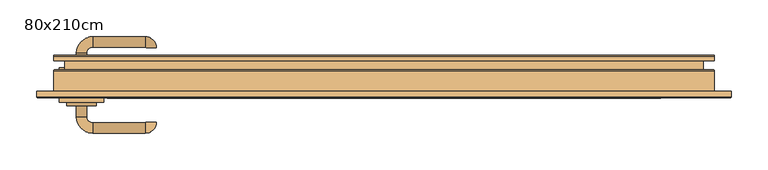
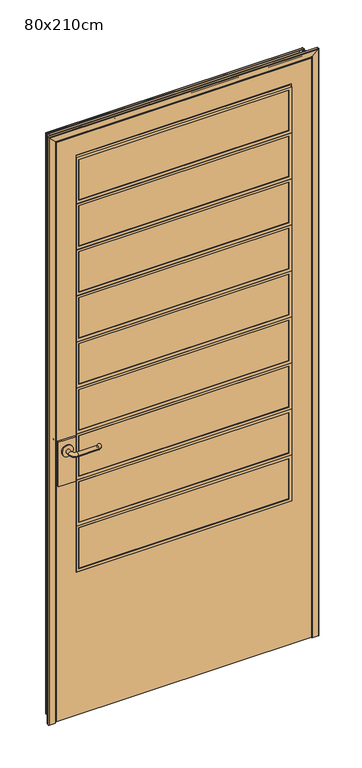
"""IFC4 building model written with IfcOpenShell, lengths in millimetres: door geometry, Porta de Abrir Metálica com Divisões Horizontais : 80x210cm."""

from ifc_helpers import new_model, si_unit, point, frame, frame_2d, origin, place, context, project, spatial, polyline, circle_curve, ellipse_curve, trimmed, segment, composite_curve, outline, extrude, source, transform, mapped, element, save
from ifc_brep_helpers import plane_surface, cylinder_surface, revolved_surface, advanced_brep


def door_80x210cm_38478dd2(model_context):
    return source(origin(), model_context, "Body", "SolidModel", [
        extrude(outline(polyline([(367.0, -87.5), (367.0, -92.5), (-367.0, -92.5), (-367.0, -87.5), (367.0, -87.5)])), frame((0.0, 0.0, 1955.6666667), z_axis=(0.0, 0.0, 1.0), x_axis=(1.0, 0.0, 0.0)), (0.0, 0.0, 1.0), 150.0),
        extrude(outline(polyline([(1945.6666667, 377.0), (2115.6666667, 377.0), (2115.6666667, -377.0), (1945.6666667, -377.0), (1945.6666667, 377.0)]), holes=[polyline([(2105.6666667, -367.0), (2105.6666667, 367.0), (1955.6666667, 367.0), (1955.6666667, -367.0), (2105.6666667, -367.0)])]), frame((0.0, -95.0, 0.0), z_axis=(0.0, 1.0, 0.0), x_axis=(0.0, 0.0, 1.0)), (0.0, 0.0, 1.0), 10.0),
        extrude(outline(polyline([(367.0, -87.5), (367.0, -92.5), (-367.0, -92.5), (-367.0, -87.5), (367.0, -87.5)])), frame((0.0, 0.0, 1785.3333333), z_axis=(0.0, 0.0, 1.0), x_axis=(1.0, 0.0, 0.0)), (0.0, 0.0, 1.0), 150.0),
        extrude(outline(polyline([(1775.3333333, 377.0), (1945.3333333, 377.0), (1945.3333333, -377.0), (1775.3333333, -377.0), (1775.3333333, 377.0)]), holes=[polyline([(1935.3333333, -367.0), (1935.3333333, 367.0), (1785.3333333, 367.0), (1785.3333333, -367.0), (1935.3333333, -367.0)])]), frame((0.0, -95.0, 0.0), z_axis=(0.0, 1.0, 0.0), x_axis=(0.0, 0.0, 1.0)), (0.0, 0.0, 1.0), 10.0),
        extrude(outline(polyline([(367.0, -87.5), (367.0, -92.5), (-367.0, -92.5), (-367.0, -87.5), (367.0, -87.5)])), frame((0.0, 0.0, 1615.0), z_axis=(0.0, 0.0, 1.0), x_axis=(1.0, 0.0, 0.0)), (0.0, 0.0, 1.0), 150.0),
        extrude(outline(polyline([(1605.0, 377.0), (1775.0, 377.0), (1775.0, -377.0), (1605.0, -377.0), (1605.0, 377.0)]), holes=[polyline([(1765.0, -367.0), (1765.0, 367.0), (1615.0, 367.0), (1615.0, -367.0), (1765.0, -367.0)])]), frame((0.0, -95.0, 0.0), z_axis=(0.0, 1.0, 0.0), x_axis=(0.0, 0.0, 1.0)), (0.0, 0.0, 1.0), 10.0),
        extrude(outline(polyline([(367.0, -87.5), (367.0, -92.5), (-367.0, -92.5), (-367.0, -87.5), (367.0, -87.5)])), frame((0.0, 0.0, 1444.6666667), z_axis=(0.0, 0.0, 1.0), x_axis=(1.0, 0.0, 0.0)), (0.0, 0.0, 1.0), 150.0),
        extrude(outline(polyline([(1434.6666667, 377.0), (1604.6666667, 377.0), (1604.6666667, -377.0), (1434.6666667, -377.0), (1434.6666667, 377.0)]), holes=[polyline([(1594.6666667, -367.0), (1594.6666667, 367.0), (1444.6666667, 367.0), (1444.6666667, -367.0), (1594.6666667, -367.0)])]), frame((0.0, -95.0, 0.0), z_axis=(0.0, 1.0, 0.0), x_axis=(0.0, 0.0, 1.0)), (0.0, 0.0, 1.0), 10.0),
        extrude(outline(polyline([(367.0, -87.5), (367.0, -92.5), (-367.0, -92.5), (-367.0, -87.5), (367.0, -87.5)])), frame((0.0, 0.0, 1274.3333333), z_axis=(0.0, 0.0, 1.0), x_axis=(1.0, 0.0, 0.0)), (0.0, 0.0, 1.0), 150.0),
        extrude(outline(polyline([(1264.3333333, 377.0), (1434.3333333, 377.0), (1434.3333333, -377.0), (1264.3333333, -377.0), (1264.3333333, 377.0)]), holes=[polyline([(1424.3333333, -367.0), (1424.3333333, 367.0), (1274.3333333, 367.0), (1274.3333333, -367.0), (1424.3333333, -367.0)])]), frame((0.0, -95.0, 0.0), z_axis=(0.0, 1.0, 0.0), x_axis=(0.0, 0.0, 1.0)), (0.0, 0.0, 1.0), 10.0),
        extrude(outline(polyline([(367.0, -87.5), (367.0, -92.5), (-367.0, -92.5), (-367.0, -87.5), (367.0, -87.5)])), frame((0.0, 0.0, 1104.0), z_axis=(0.0, 0.0, 1.0), x_axis=(1.0, 0.0, 0.0)), (0.0, 0.0, 1.0), 150.0),
        extrude(outline(polyline([(1094.0, 377.0), (1264.0, 377.0), (1264.0, -377.0), (1094.0, -377.0), (1094.0, 377.0)]), holes=[polyline([(1254.0, -367.0), (1254.0, 367.0), (1104.0, 367.0), (1104.0, -367.0), (1254.0, -367.0)])]), frame((0.0, -95.0, 0.0), z_axis=(0.0, 1.0, 0.0), x_axis=(0.0, 0.0, 1.0)), (0.0, 0.0, 1.0), 10.0),
        extrude(outline(polyline([(367.0, -87.5), (367.0, -92.5), (-367.0, -92.5), (-367.0, -87.5), (367.0, -87.5)])), frame((0.0, 0.0, 933.6666667), z_axis=(0.0, 0.0, 1.0), x_axis=(1.0, 0.0, 0.0)), (0.0, 0.0, 1.0), 150.0),
        extrude(outline(polyline([(923.6666667, 377.0), (1093.6666667, 377.0), (1093.6666667, -377.0), (923.6666667, -377.0), (923.6666667, 377.0)]), holes=[polyline([(1083.6666667, -367.0), (1083.6666667, 367.0), (933.6666667, 367.0), (933.6666667, -367.0), (1083.6666667, -367.0)])]), frame((0.0, -95.0, 0.0), z_axis=(0.0, 1.0, 0.0), x_axis=(0.0, 0.0, 1.0)), (0.0, 0.0, 1.0), 10.0),
        extrude(outline(polyline([(367.0, -87.5), (367.0, -92.5), (-367.0, -92.5), (-367.0, -87.5), (367.0, -87.5)])), frame((0.0, 0.0, 763.3333333), z_axis=(0.0, 0.0, 1.0), x_axis=(1.0, 0.0, 0.0)), (0.0, 0.0, 1.0), 150.0),
        extrude(outline(polyline([(753.3333333, 377.0), (923.3333333, 377.0), (923.3333333, -377.0), (753.3333333, -377.0), (753.3333333, 377.0)]), holes=[polyline([(913.3333333, -367.0), (913.3333333, 367.0), (763.3333333, 367.0), (763.3333333, -367.0), (913.3333333, -367.0)])]), frame((0.0, -95.0, 0.0), z_axis=(0.0, 1.0, 0.0), x_axis=(0.0, 0.0, 1.0)), (0.0, 0.0, 1.0), 10.0),
        extrude(outline(polyline([(367.0, -87.5), (367.0, -92.5), (-367.0, -92.5), (-367.0, -87.5), (367.0, -87.5)])), frame((0.0, 0.0, 593.0), z_axis=(0.0, 0.0, 1.0), x_axis=(1.0, 0.0, 0.0)), (0.0, 0.0, 1.0), 150.0),
        extrude(outline(polyline([(583.0, 377.0), (753.0, 377.0), (753.0, -377.0), (583.0, -377.0), (583.0, 377.0)]), holes=[polyline([(743.0, -367.0), (743.0, 367.0), (593.0, 367.0), (593.0, -367.0), (743.0, -367.0)])]), frame((0.0, -95.0, 0.0), z_axis=(0.0, 1.0, 0.0), x_axis=(0.0, 0.0, 1.0)), (0.0, 0.0, 1.0), 10.0),
        extrude(outline(composite_curve([segment(trimmed(circle_curve(frame_2d((1050.0, -412.0)), 20.0), [point((1050.0, -432.0))], [point((1050.0, -392.0))], False, "CARTESIAN"), True, "CONTINUOUS"), segment(trimmed(circle_curve(frame_2d((1050.0, -412.0)), 20.0), [point((1050.0, -392.0))], [point((1050.0, -432.0))], False, "CARTESIAN"), True, "CONTINUOUS")], self_intersect=False)), frame((0.0, -53.6, 0.0), z_axis=(0.0, 1.0, 0.0), x_axis=(0.0, 0.0, 1.0)), (0.0, 0.0, 1.0), 4.5929895),
        advanced_brep(
        [(-405.0, -49.0070105, 1050.0), (-419.0, -49.0070105, 1050.0), (-405.0, -33.6, 1050.0), (-419.0, -33.6, 1050.0), (-397.0, -11.6, 1050.0), (-397.0, -25.6, 1050.0), (-325.0, -25.6, 1050.0), (-325.0, -11.6, 1050.0), (-324.0, -26.6, 1050.0), (-310.0, -26.6, 1050.0)],
        [
            (0, 1, circle_curve(frame((-412.0, -49.0070105, 1050.0), z_axis=(0.0, -1.0, 0.0), x_axis=(-1.0, 0.0, 0.0)), 7.0)),
            (1, 0, circle_curve(frame((-412.0, -49.0070105, 1050.0), z_axis=(0.0, -1.0, 0.0), x_axis=(-1.0, 0.0, 0.0)), 7.0)),
            (0, 2),
            (2, 3, circle_curve(frame((-412.0, -33.6, 1050.0), z_axis=(0.0, -1.0, 0.0), x_axis=(-1.0, 0.0, 0.0)), 7.0)),
            (3, 1),
            (3, 2, circle_curve(frame((-412.0, -33.6, 1050.0), z_axis=(0.0, -1.0, 0.0), x_axis=(-1.0, 0.0, 0.0)), 7.0)),
            (4, 3, circle_curve(frame((-397.0, -33.6, 1050.0), z_axis=(0.0, 0.0, 1.0), x_axis=(-1.0, 0.0, 0.0)), 22.0)),
            (2, 5, circle_curve(frame((-397.0, -33.6, 1050.0), z_axis=(0.0, 0.0, -1.0), x_axis=(-1.0, 0.0, 0.0)), 8.0)),
            (5, 4, circle_curve(frame((-397.0, -18.6, 1050.0), z_axis=(-1.0, 0.0, 0.0), x_axis=(0.0, 1.0, 0.0)), 7.0)),
            (4, 5, circle_curve(frame((-397.0, -18.6, 1050.0), z_axis=(-1.0, 0.0, 0.0), x_axis=(0.0, 1.0, 0.0)), 7.0)),
            (5, 6),
            (6, 7, circle_curve(frame((-325.0, -18.6, 1050.0), z_axis=(-1.0, 0.0, 0.0), x_axis=(0.0, 1.0, 0.0)), 7.0)),
            (7, 4),
            (7, 6, circle_curve(frame((-325.0, -18.6, 1050.0), z_axis=(-1.0, 0.0, 0.0), x_axis=(0.0, 1.0, 0.0)), 7.0)),
            (8, 9, circle_curve(frame((-317.0, -26.6, 1050.0), z_axis=(0.0, -1.0, 0.0), x_axis=(1.0, 0.0, 0.0)), 7.0)),
            (9, 8, circle_curve(frame((-317.0, -26.6, 1050.0), z_axis=(0.0, -1.0, 0.0), x_axis=(1.0, 0.0, 0.0)), 7.0)),
            (9, 7, circle_curve(frame((-325.0, -26.6, 1050.0), z_axis=(0.0, 0.0, 1.0), x_axis=(0.0, 1.0, 0.0)), 15.0)),
            (6, 8, circle_curve(frame((-325.0, -26.6, 1050.0), z_axis=(0.0, 0.0, -1.0), x_axis=(0.0, 1.0, 0.0)), 1.0)),
        ],
        [
            plane_surface(frame((-412.0, -49.0070105, 1050.0), z_axis=(0.0, -1.0, 0.0), x_axis=(0.0, 0.0, 1.0))),
            cylinder_surface(frame((-412.0, -49.0070105, 1050.0), z_axis=(0.0, -1.0, 0.0), x_axis=(-1.0, 0.0, 0.0)), 7.0),
            revolved_surface(trimmed(ellipse_curve(frame((-412.0, -33.6, 1050.0), z_axis=(0.0, -1.0, 0.0), x_axis=(-1.0, 0.0, 0.0)), 7.0, 7.0), [point((-405.0, -33.6, 1050.0))], [point((-419.0, -33.6, 1050.0))], True, "CARTESIAN"), (-397.0, -33.6, 1050.0), (0.0, 0.0, -1.0)),
            revolved_surface(trimmed(ellipse_curve(frame((-412.0, -33.6, 1050.0), z_axis=(0.0, -1.0, 0.0), x_axis=(-1.0, 0.0, 0.0)), 7.0, 7.0), [point((-419.0, -33.6, 1050.0))], [point((-405.0, -33.6, 1050.0))], True, "CARTESIAN"), (-397.0, -33.6, 1050.0), (0.0, 0.0, -1.0)),
            cylinder_surface(frame((-397.0, -18.6, 1050.0), z_axis=(-1.0, 0.0, 0.0), x_axis=(0.0, 1.0, 0.0)), 7.0),
            plane_surface(frame((-317.0, -26.6, 1050.0), z_axis=(0.0, -1.0, 0.0), x_axis=(0.0, 0.0, 1.0))),
            revolved_surface(trimmed(ellipse_curve(frame((-325.0, -18.6, 1050.0), z_axis=(-1.0, 0.0, 0.0), x_axis=(0.0, 1.0, 0.0)), 7.0, 7.0), [point((-325.0, -25.6, 1050.0))], [point((-325.0, -11.6, 1050.0))], True, "CARTESIAN"), (-325.0, -26.6, 1050.0), (0.0, 0.0, -1.0)),
            revolved_surface(trimmed(ellipse_curve(frame((-325.0, -18.6, 1050.0), z_axis=(-1.0, 0.0, 0.0), x_axis=(0.0, 1.0, 0.0)), 7.0, 7.0), [point((-325.0, -11.6, 1050.0))], [point((-325.0, -25.6, 1050.0))], True, "CARTESIAN"), (-325.0, -26.6, 1050.0), (0.0, 0.0, -1.0)),
        ],
        [
            (0, [[1, 2]]),
            (1, [[-1, 3, 4, 5]]),
            (1, [[-2, -5, 6, -3]]),
            (2, [[7, -4, 8, 9]]),
            (3, [[-8, -6, -7, 10]]),
            (4, [[-9, 11, 12, 13]]),
            (4, [[-10, -13, 14, -11]]),
            (5, [[15, 16]]),
            (6, [[17, -12, 18, -16]]),
            (7, [[-18, -14, -17, -15]]),
        ],
    ),
        extrude(outline(polyline([(-382.0, -59.6), (-442.0, -59.6), (-442.0, -53.6), (-382.0, -53.6), (-382.0, -59.6)])), frame((0.0, 0.0, 925.0), z_axis=(0.0, 0.0, 1.0), x_axis=(1.0, 0.0, 0.0)), (0.0, 0.0, 1.0), 165.0),
        extrude(outline(composite_curve([segment(trimmed(circle_curve(frame_2d((1050.0, -412.0)), 20.0), [point((1050.0, -432.0))], [point((1050.0, -392.0))], False, "CARTESIAN"), True, "CONTINUOUS"), segment(trimmed(circle_curve(frame_2d((1050.0, -412.0)), 20.0), [point((1050.0, -392.0))], [point((1050.0, -432.0))], False, "CARTESIAN"), True, "CONTINUOUS")], self_intersect=False)), frame((0.0, -105.1929895, 0.0), z_axis=(0.0, 1.0, 0.0), x_axis=(0.0, 0.0, 1.0)), (0.0, 0.0, 1.0), 4.5929895),
        advanced_brep(
        [(-405.0, -105.1929895, 1050.0), (-419.0, -105.1929895, 1050.0), (-419.0, -120.6, 1050.0), (-405.0, -120.6, 1050.0), (-397.0, -142.6, 1050.0), (-397.0, -128.6, 1050.0), (-325.0, -142.6, 1050.0), (-325.0, -128.6, 1050.0), (-324.0, -127.6, 1050.0), (-310.0, -127.6, 1050.0)],
        [
            (0, 1, circle_curve(frame((-412.0, -105.1929895, 1050.0), z_axis=(0.0, 1.0, 0.0), x_axis=(-1.0, 0.0, 0.0)), 7.0)),
            (1, 0, circle_curve(frame((-412.0, -105.1929895, 1050.0), z_axis=(0.0, 1.0, 0.0), x_axis=(-1.0, 0.0, 0.0)), 7.0)),
            (1, 2),
            (2, 3, circle_curve(frame((-412.0, -120.6, 1050.0), z_axis=(0.0, 1.0, 0.0), x_axis=(-1.0, 0.0, 0.0)), 7.0)),
            (3, 0),
            (3, 2, circle_curve(frame((-412.0, -120.6, 1050.0), z_axis=(0.0, 1.0, 0.0), x_axis=(-1.0, 0.0, 0.0)), 7.0)),
            (4, 5, circle_curve(frame((-397.0, -135.6, 1050.0), z_axis=(-1.0, 0.0, 0.0), x_axis=(0.0, -1.0, 0.0)), 7.0)),
            (5, 3, circle_curve(frame((-397.0, -120.6, 1050.0), z_axis=(0.0, 0.0, -1.0), x_axis=(-1.0, 0.0, 0.0)), 8.0)),
            (2, 4, circle_curve(frame((-397.0, -120.6, 1050.0), z_axis=(0.0, 0.0, 1.0), x_axis=(-1.0, 0.0, 0.0)), 22.0)),
            (5, 4, circle_curve(frame((-397.0, -135.6, 1050.0), z_axis=(-1.0, 0.0, 0.0), x_axis=(0.0, -1.0, 0.0)), 7.0)),
            (4, 6),
            (6, 7, circle_curve(frame((-325.0, -135.6, 1050.0), z_axis=(-1.0, 0.0, 0.0), x_axis=(0.0, -1.0, 0.0)), 7.0)),
            (7, 5),
            (7, 6, circle_curve(frame((-325.0, -135.6, 1050.0), z_axis=(-1.0, 0.0, 0.0), x_axis=(0.0, -1.0, 0.0)), 7.0)),
            (8, 9, circle_curve(frame((-317.0, -127.6, 1050.0), z_axis=(0.0, 1.0, 0.0), x_axis=(1.0, 0.0, 0.0)), 7.0)),
            (9, 8, circle_curve(frame((-317.0, -127.6, 1050.0), z_axis=(0.0, 1.0, 0.0), x_axis=(1.0, 0.0, 0.0)), 7.0)),
            (8, 7, circle_curve(frame((-325.0, -127.6, 1050.0), z_axis=(0.0, 0.0, -1.0), x_axis=(0.0, -1.0, 0.0)), 1.0)),
            (6, 9, circle_curve(frame((-325.0, -127.6, 1050.0), z_axis=(0.0, 0.0, 1.0), x_axis=(0.0, -1.0, 0.0)), 15.0)),
        ],
        [
            plane_surface(frame((-412.0, -105.1929895, 1050.0), z_axis=(0.0, 1.0, 0.0), x_axis=(0.0, 0.0, 1.0))),
            cylinder_surface(frame((-412.0, -105.1929895, 1050.0), z_axis=(0.0, 1.0, 0.0), x_axis=(-1.0, 0.0, 0.0)), 7.0),
            revolved_surface(trimmed(ellipse_curve(frame((-412.0, -120.6, 1050.0), z_axis=(0.0, -1.0, 0.0), x_axis=(-1.0, 0.0, 0.0)), 7.0, 7.0), [point((-405.0, -120.6, 1050.0))], [point((-419.0, -120.6, 1050.0))], True, "CARTESIAN"), (-397.0, -120.6, 1050.0), (0.0, 0.0, -1.0)),
            revolved_surface(trimmed(ellipse_curve(frame((-412.0, -120.6, 1050.0), z_axis=(0.0, -1.0, 0.0), x_axis=(-1.0, 0.0, 0.0)), 7.0, 7.0), [point((-419.0, -120.6, 1050.0))], [point((-405.0, -120.6, 1050.0))], True, "CARTESIAN"), (-397.0, -120.6, 1050.0), (0.0, 0.0, -1.0)),
            cylinder_surface(frame((-397.0, -135.6, 1050.0), z_axis=(-1.0, 0.0, 0.0), x_axis=(0.0, -1.0, 0.0)), 7.0),
            plane_surface(frame((-317.0, -127.6, 1050.0), z_axis=(0.0, 1.0, 0.0), x_axis=(0.0, 0.0, 1.0))),
            revolved_surface(trimmed(ellipse_curve(frame((-325.0, -135.6, 1050.0), z_axis=(1.0, 0.0, 0.0), x_axis=(0.0, -1.0, 0.0)), 7.0, 7.0), [point((-325.0, -128.6, 1050.0))], [point((-325.0, -142.6, 1050.0))], True, "CARTESIAN"), (-325.0, -127.6, 1050.0), (0.0, 0.0, -1.0)),
            revolved_surface(trimmed(ellipse_curve(frame((-325.0, -135.6, 1050.0), z_axis=(1.0, 0.0, 0.0), x_axis=(0.0, -1.0, 0.0)), 7.0, 7.0), [point((-325.0, -142.6, 1050.0))], [point((-325.0, -128.6, 1050.0))], True, "CARTESIAN"), (-325.0, -127.6, 1050.0), (0.0, 0.0, -1.0)),
        ],
        [
            (0, [[1, 2]]),
            (1, [[3, 4, 5, -2]]),
            (1, [[-5, 6, -3, -1]]),
            (2, [[7, 8, -4, 9]]),
            (3, [[10, -9, -6, -8]]),
            (4, [[11, 12, 13, -7]]),
            (4, [[-13, 14, -11, -10]]),
            (5, [[15, 16]]),
            (6, [[-15, 17, -12, 18]]),
            (7, [[-16, -18, -14, -17]]),
        ],
    ),
        extrude(outline(polyline([(-382.0, -94.6), (-382.0, -100.6), (-442.0, -100.6), (-442.0, -94.6), (-382.0, -94.6)])), frame((0.0, 0.0, 925.0), z_axis=(0.0, 0.0, 1.0), x_axis=(1.0, 0.0, 0.0)), (0.0, 0.0, 1.0), 165.0),
        extrude(outline(polyline([(2196.0, -447.0), (53.0, -447.0), (53.0, 447.0), (2196.0, 447.0), (2196.0, -447.0)]), holes=[polyline([(2126.0, -377.0), (2126.0, 377.0), (583.0, 377.0), (583.0, -377.0), (2126.0, -377.0)])]), frame((0.0, -94.6, 0.0), z_axis=(0.0, 1.0, 0.0), x_axis=(0.0, 0.0, 1.0)), (0.0, 0.0, 1.0), 35.0),
        advanced_brep(
        [(-435.45, -36.6755478, 50.0), (-433.95, -38.1755478, 50.0), (-433.95, -56.1755478, 50.0), (-435.45, -57.6755478, 50.0), (-448.5, -57.6755478, 50.0), (-449.0, -58.1755478, 50.0), (-449.0, -93.1755478, 50.0), (-450.5, -94.6755478, 50.0), (-471.5, -94.6755478, 50.0), (-473.0, -93.1755478, 50.0), (-473.0, -85.6755478, 50.0), (-472.0, -85.6755478, 50.0), (-472.0, -93.1755478, 50.0), (-471.5, -93.6755478, 50.0), (-450.5, -93.6755478, 50.0), (-450.0, -93.1755478, 50.0), (-450.0, -58.1755478, 50.0), (-448.5, -56.6755478, 50.0), (-435.45, -56.6755478, 50.0), (-434.95, -56.1755478, 50.0), (-434.95, -38.1755478, 50.0), (-435.45, -37.6755478, 50.0), (-448.45, -37.6755478, 50.0), (-448.95, -38.1755478, 50.0), (-448.95, -44.6755478, 50.0), (-449.95, -44.6755478, 50.0), (-449.95, -38.1755478, 50.0), (-448.45, -36.6755478, 50.0), (435.45, -36.6755478, 50.0), (448.45, -36.6755478, 50.0), (449.95, -38.1755478, 50.0), (449.95, -44.6755478, 50.0), (448.95, -44.6755478, 50.0), (448.95, -38.1755478, 50.0), (448.45, -37.6755478, 50.0), (435.45, -37.6755478, 50.0), (434.95, -38.1755478, 50.0), (434.95, -56.1755478, 50.0), (435.45, -56.6755478, 50.0), (448.5, -56.6755478, 50.0), (450.0, -58.1755478, 50.0), (450.0, -93.1755478, 50.0), (450.5, -93.6755478, 50.0), (471.5, -93.6755478, 50.0), (472.0, -93.1755478, 50.0), (472.0, -85.6755478, 50.0), (473.0, -85.6755478, 50.0), (473.0, -93.1755478, 50.0), (471.5, -94.6755478, 50.0), (450.5, -94.6755478, 50.0), (449.0, -93.1755478, 50.0), (449.0, -58.1755478, 50.0), (448.5, -57.6755478, 50.0), (435.45, -57.6755478, 50.0), (433.95, -56.1755478, 50.0), (433.95, -38.1755478, 50.0), (-448.45, -36.6755478, 2198.45), (-435.45, -36.6755478, 2185.45), (-449.95, -38.1755478, 2199.95), (-449.95, -44.6755478, 2199.95), (-448.95, -44.6755478, 2198.95), (-448.95, -38.1755478, 2198.95), (-448.45, -37.6755478, 2198.45), (-435.45, -37.6755478, 2185.45), (-434.95, -38.1755478, 2184.95), (-434.95, -56.1755478, 2184.95), (-435.45, -56.6755478, 2185.45), (-448.5, -56.6755478, 2198.5), (-450.0, -58.1755478, 2200.0), (-450.0, -93.1755478, 2200.0), (-450.5, -93.6755478, 2200.5), (-471.5, -93.6755478, 2221.5), (-472.0, -93.1755478, 2222.0), (-472.0, -85.6755478, 2222.0), (-473.0, -85.6755478, 2223.0), (-473.0, -93.1755478, 2223.0), (-471.5, -94.6755478, 2221.5), (-450.5, -94.6755478, 2200.5), (-449.0, -93.1755478, 2199.0), (-449.0, -58.1755478, 2199.0), (-448.5, -57.6755478, 2198.5), (-435.45, -57.6755478, 2185.45), (-433.95, -56.1755478, 2183.95), (-433.95, -38.1755478, 2183.95), (435.45, -36.6755478, 2185.45), (433.95, -38.1755478, 2183.95), (433.95, -56.1755478, 2183.95), (435.45, -57.6755478, 2185.45), (448.5, -57.6755478, 2198.5), (449.0, -58.1755478, 2199.0), (449.0, -93.1755478, 2199.0), (450.5, -94.6755478, 2200.5), (471.5, -94.6755478, 2221.5), (473.0, -93.1755478, 2223.0), (473.0, -85.6755478, 2223.0), (472.0, -85.6755478, 2222.0), (472.0, -93.1755478, 2222.0), (471.5, -93.6755478, 2221.5), (450.5, -93.6755478, 2200.5), (450.0, -93.1755478, 2200.0), (450.0, -58.1755478, 2200.0), (448.5, -56.6755478, 2198.5), (435.45, -56.6755478, 2185.45), (434.95, -56.1755478, 2184.95), (434.95, -38.1755478, 2184.95), (435.45, -37.6755478, 2185.45), (448.45, -37.6755478, 2198.45), (448.95, -38.1755478, 2198.95), (448.95, -44.6755478, 2198.95), (449.95, -44.6755478, 2199.95), (449.95, -38.1755478, 2199.95), (448.45, -36.6755478, 2198.45)],
        [
            (0, 1, circle_curve(frame((-435.45, -38.1755478, 50.0), z_axis=(0.0, 0.0, -1.0), x_axis=(1.0, 0.0, 0.0)), 1.5)),
            (1, 2),
            (2, 3, circle_curve(frame((-435.45, -56.1755478, 50.0), z_axis=(0.0, 0.0, -1.0), x_axis=(1.0, 0.0, 0.0)), 1.5)),
            (3, 4),
            (4, 5, circle_curve(frame((-448.5, -58.1755478, 50.0), z_axis=(0.0, 0.0, 1.0), x_axis=(1.0, 0.0, 0.0)), 0.5)),
            (5, 6),
            (6, 7, circle_curve(frame((-450.5, -93.1755478, 50.0), z_axis=(0.0, 0.0, -1.0), x_axis=(1.0, 0.0, 0.0)), 1.5)),
            (7, 8),
            (8, 9, circle_curve(frame((-471.5, -93.1755478, 50.0), z_axis=(0.0, 0.0, -1.0), x_axis=(1.0, 0.0, 0.0)), 1.5)),
            (9, 10),
            (10, 11),
            (11, 12),
            (12, 13, circle_curve(frame((-471.5, -93.1755478, 50.0), z_axis=(0.0, 0.0, 1.0), x_axis=(1.0, 0.0, 0.0)), 0.5)),
            (13, 14),
            (14, 15, circle_curve(frame((-450.5, -93.1755478, 50.0), z_axis=(0.0, 0.0, 1.0), x_axis=(1.0, 0.0, 0.0)), 0.5)),
            (15, 16),
            (16, 17, circle_curve(frame((-448.5, -58.1755478, 50.0), z_axis=(0.0, 0.0, -1.0), x_axis=(1.0, 0.0, 0.0)), 1.5)),
            (17, 18),
            (18, 19, circle_curve(frame((-435.45, -56.1755478, 50.0), z_axis=(0.0, 0.0, 1.0), x_axis=(1.0, 0.0, 0.0)), 0.5)),
            (19, 20),
            (20, 21, circle_curve(frame((-435.45, -38.1755478, 50.0), z_axis=(0.0, 0.0, 1.0), x_axis=(1.0, 0.0, 0.0)), 0.5)),
            (21, 22),
            (22, 23, circle_curve(frame((-448.45, -38.1755478, 50.0), z_axis=(0.0, 0.0, 1.0), x_axis=(1.0, 0.0, 0.0)), 0.5)),
            (23, 24),
            (24, 25),
            (25, 26),
            (26, 27, circle_curve(frame((-448.45, -38.1755478, 50.0), z_axis=(0.0, 0.0, -1.0), x_axis=(1.0, 0.0, 0.0)), 1.5)),
            (27, 0),
            (28, 29),
            (29, 30, circle_curve(frame((448.45, -38.1755478, 50.0), z_axis=(0.0, 0.0, -1.0), x_axis=(-1.0, 0.0, 0.0)), 1.5)),
            (30, 31),
            (31, 32),
            (32, 33),
            (33, 34, circle_curve(frame((448.45, -38.1755478, 50.0), z_axis=(0.0, 0.0, 1.0), x_axis=(-1.0, 0.0, 0.0)), 0.5)),
            (34, 35),
            (35, 36, circle_curve(frame((435.45, -38.1755478, 50.0), z_axis=(0.0, 0.0, 1.0), x_axis=(-1.0, 0.0, 0.0)), 0.5)),
            (36, 37),
            (37, 38, circle_curve(frame((435.45, -56.1755478, 50.0), z_axis=(0.0, 0.0, 1.0), x_axis=(-1.0, 0.0, 0.0)), 0.5)),
            (38, 39),
            (39, 40, circle_curve(frame((448.5, -58.1755478, 50.0), z_axis=(0.0, 0.0, -1.0), x_axis=(-1.0, 0.0, 0.0)), 1.5)),
            (40, 41),
            (41, 42, circle_curve(frame((450.5, -93.1755478, 50.0), z_axis=(0.0, 0.0, 1.0), x_axis=(-1.0, 0.0, 0.0)), 0.5)),
            (42, 43),
            (43, 44, circle_curve(frame((471.5, -93.1755478, 50.0), z_axis=(0.0, 0.0, 1.0), x_axis=(-1.0, 0.0, 0.0)), 0.5)),
            (44, 45),
            (45, 46),
            (46, 47),
            (47, 48, circle_curve(frame((471.5, -93.1755478, 50.0), z_axis=(0.0, 0.0, -1.0), x_axis=(-1.0, 0.0, 0.0)), 1.5)),
            (48, 49),
            (49, 50, circle_curve(frame((450.5, -93.1755478, 50.0), z_axis=(0.0, 0.0, -1.0), x_axis=(-1.0, 0.0, 0.0)), 1.5)),
            (50, 51),
            (51, 52, circle_curve(frame((448.5, -58.1755478, 50.0), z_axis=(0.0, 0.0, 1.0), x_axis=(-1.0, 0.0, 0.0)), 0.5)),
            (52, 53),
            (53, 54, circle_curve(frame((435.45, -56.1755478, 50.0), z_axis=(0.0, 0.0, -1.0), x_axis=(-1.0, 0.0, 0.0)), 1.5)),
            (54, 55),
            (55, 28, circle_curve(frame((435.45, -38.1755478, 50.0), z_axis=(0.0, 0.0, -1.0), x_axis=(-1.0, 0.0, 0.0)), 1.5)),
            (27, 56),
            (56, 57),
            (57, 0),
            (26, 58),
            (58, 56, ellipse_curve(frame((-448.45, -38.1755478, 2198.45), z_axis=(-0.7071067811865475, 0.0, -0.7071067811865475), x_axis=(0.7071067811865474, 0.0, -0.7071067811865476)), 2.1213203, 1.5)),
            (25, 59),
            (59, 58),
            (24, 60),
            (60, 59),
            (23, 61),
            (61, 60),
            (22, 62),
            (62, 61, ellipse_curve(frame((-448.45, -38.1755478, 2198.45), z_axis=(0.7071067811865475, 0.0, 0.7071067811865475), x_axis=(-0.7071067811865474, 0.0, 0.7071067811865476)), 0.7071068, 0.5)),
            (21, 63),
            (63, 62),
            (20, 64),
            (64, 63, ellipse_curve(frame((-435.45, -38.1755478, 2185.45), z_axis=(0.7071067811865475, 0.0, 0.7071067811865475), x_axis=(-0.7071067811865474, 0.0, 0.7071067811865476)), 0.7071068, 0.5)),
            (19, 65),
            (65, 64),
            (18, 66),
            (66, 65, ellipse_curve(frame((-435.45, -56.1755478, 2185.45), z_axis=(0.7071067811865475, 0.0, 0.7071067811865475), x_axis=(-0.7071067811865474, 0.0, 0.7071067811865476)), 0.7071068, 0.5)),
            (17, 67),
            (67, 66),
            (16, 68),
            (68, 67, ellipse_curve(frame((-448.5, -58.1755478, 2198.5), z_axis=(-0.7071067811865475, 0.0, -0.7071067811865475), x_axis=(0.7071067811865474, 0.0, -0.7071067811865476)), 2.1213203, 1.5)),
            (15, 69),
            (69, 68),
            (14, 70),
            (70, 69, ellipse_curve(frame((-450.5, -93.1755478, 2200.5), z_axis=(0.7071067811865475, 0.0, 0.7071067811865475), x_axis=(-0.7071067811865474, 0.0, 0.7071067811865476)), 0.7071068, 0.5)),
            (13, 71),
            (71, 70),
            (12, 72),
            (72, 71, ellipse_curve(frame((-471.5, -93.1755478, 2221.5), z_axis=(0.7071067811865475, 0.0, 0.7071067811865475), x_axis=(-0.7071067811865474, 0.0, 0.7071067811865476)), 0.7071068, 0.5)),
            (11, 73),
            (73, 72),
            (10, 74),
            (74, 73),
            (9, 75),
            (75, 74),
            (8, 76),
            (76, 75, ellipse_curve(frame((-471.5, -93.1755478, 2221.5), z_axis=(-0.7071067811865475, 0.0, -0.7071067811865475), x_axis=(0.7071067811865474, 0.0, -0.7071067811865476)), 2.1213203, 1.5)),
            (7, 77),
            (77, 76),
            (6, 78),
            (78, 77, ellipse_curve(frame((-450.5, -93.1755478, 2200.5), z_axis=(-0.7071067811865475, 0.0, -0.7071067811865475), x_axis=(0.7071067811865474, 0.0, -0.7071067811865476)), 2.1213203, 1.5)),
            (5, 79),
            (79, 78),
            (4, 80),
            (80, 79, ellipse_curve(frame((-448.5, -58.1755478, 2198.5), z_axis=(0.7071067811865475, 0.0, 0.7071067811865475), x_axis=(-0.7071067811865474, 0.0, 0.7071067811865476)), 0.7071068, 0.5)),
            (3, 81),
            (81, 80),
            (2, 82),
            (82, 81, ellipse_curve(frame((-435.45, -56.1755478, 2185.45), z_axis=(-0.7071067811865475, 0.0, -0.7071067811865475), x_axis=(0.7071067811865474, 0.0, -0.7071067811865476)), 2.1213203, 1.5)),
            (1, 83),
            (83, 82),
            (57, 83, ellipse_curve(frame((-435.45, -38.1755478, 2185.45), z_axis=(-0.7071067811865475, 0.0, -0.7071067811865475), x_axis=(0.7071067811865474, 0.0, -0.7071067811865476)), 2.1213203, 1.5)),
            (84, 28),
            (55, 85),
            (85, 84, ellipse_curve(frame((435.45, -38.1755478, 2185.45), z_axis=(0.7071067811865475, 0.0, -0.7071067811865475), x_axis=(0.7071067811865474, 0.0, 0.7071067811865476)), 2.1213203, 1.5)),
            (54, 86),
            (86, 85),
            (53, 87),
            (87, 86, ellipse_curve(frame((435.45, -56.1755478, 2185.45), z_axis=(0.7071067811865475, 0.0, -0.7071067811865475), x_axis=(0.7071067811865474, 0.0, 0.7071067811865476)), 2.1213203, 1.5)),
            (52, 88),
            (88, 87),
            (51, 89),
            (89, 88, ellipse_curve(frame((448.5, -58.1755478, 2198.5), z_axis=(-0.7071067811865475, 0.0, 0.7071067811865475), x_axis=(-0.7071067811865474, 0.0, -0.7071067811865476)), 0.7071068, 0.5)),
            (50, 90),
            (90, 89),
            (49, 91),
            (91, 90, ellipse_curve(frame((450.5, -93.1755478, 2200.5), z_axis=(0.7071067811865475, 0.0, -0.7071067811865475), x_axis=(0.7071067811865474, 0.0, 0.7071067811865476)), 2.1213203, 1.5)),
            (48, 92),
            (92, 91),
            (47, 93),
            (93, 92, ellipse_curve(frame((471.5, -93.1755478, 2221.5), z_axis=(0.7071067811865475, 0.0, -0.7071067811865475), x_axis=(0.7071067811865474, 0.0, 0.7071067811865476)), 2.1213203, 1.5)),
            (46, 94),
            (94, 93),
            (45, 95),
            (95, 94),
            (44, 96),
            (96, 95),
            (43, 97),
            (97, 96, ellipse_curve(frame((471.5, -93.1755478, 2221.5), z_axis=(-0.7071067811865475, 0.0, 0.7071067811865475), x_axis=(-0.7071067811865474, 0.0, -0.7071067811865476)), 0.7071068, 0.5)),
            (42, 98),
            (98, 97),
            (41, 99),
            (99, 98, ellipse_curve(frame((450.5, -93.1755478, 2200.5), z_axis=(-0.7071067811865475, 0.0, 0.7071067811865475), x_axis=(-0.7071067811865474, 0.0, -0.7071067811865476)), 0.7071068, 0.5)),
            (40, 100),
            (100, 99),
            (39, 101),
            (101, 100, ellipse_curve(frame((448.5, -58.1755478, 2198.5), z_axis=(0.7071067811865475, 0.0, -0.7071067811865475), x_axis=(0.7071067811865474, 0.0, 0.7071067811865476)), 2.1213203, 1.5)),
            (38, 102),
            (102, 101),
            (37, 103),
            (103, 102, ellipse_curve(frame((435.45, -56.1755478, 2185.45), z_axis=(-0.7071067811865475, 0.0, 0.7071067811865475), x_axis=(-0.7071067811865474, 0.0, -0.7071067811865476)), 0.7071068, 0.5)),
            (36, 104),
            (104, 103),
            (35, 105),
            (105, 104, ellipse_curve(frame((435.45, -38.1755478, 2185.45), z_axis=(-0.7071067811865475, 0.0, 0.7071067811865475), x_axis=(-0.7071067811865474, 0.0, -0.7071067811865476)), 0.7071068, 0.5)),
            (34, 106),
            (106, 105),
            (33, 107),
            (107, 106, ellipse_curve(frame((448.45, -38.1755478, 2198.45), z_axis=(-0.7071067811865475, 0.0, 0.7071067811865475), x_axis=(-0.7071067811865474, 0.0, -0.7071067811865476)), 0.7071068, 0.5)),
            (32, 108),
            (108, 107),
            (31, 109),
            (109, 108),
            (30, 110),
            (110, 109),
            (29, 111),
            (111, 110, ellipse_curve(frame((448.45, -38.1755478, 2198.45), z_axis=(0.7071067811865475, 0.0, -0.7071067811865475), x_axis=(0.7071067811865474, 0.0, 0.7071067811865476)), 2.1213203, 1.5)),
            (84, 111),
            (56, 111),
            (84, 57),
            (58, 110),
            (59, 109),
            (60, 108),
            (61, 107),
            (62, 106),
            (63, 105),
            (64, 104),
            (65, 103),
            (66, 102),
            (67, 101),
            (68, 100),
            (69, 99),
            (70, 98),
            (71, 97),
            (72, 96),
            (73, 95),
            (74, 94),
            (75, 93),
            (76, 92),
            (77, 91),
            (78, 90),
            (79, 89),
            (80, 88),
            (81, 87),
            (82, 86),
            (83, 85),
        ],
        [
            plane_surface(frame((-450.0, -34.5578163, 50.0), z_axis=(0.0, 0.0, -1.0), x_axis=(1.0, 0.0, 0.0))),
            plane_surface(frame((450.0, -34.5578163, 50.0), z_axis=(0.0, 0.0, -1.0), x_axis=(-1.0, 0.0, 0.0))),
            plane_surface(frame((-435.45, -36.6755478, 50.0), z_axis=(0.0, 1.0, 0.0), x_axis=(0.0, 0.0, 1.0))),
            cylinder_surface(frame((-448.45, -38.1755478, 50.0), z_axis=(0.0, 0.0, -1.0), x_axis=(1.0, 0.0, 0.0)), 1.5),
            plane_surface(frame((-449.95, -38.1755478, 50.0), z_axis=(-1.0, 0.0, 0.0), x_axis=(0.0, 0.0, 1.0))),
            plane_surface(frame((-449.95, -44.6755478, 50.0), z_axis=(0.0, -1.0, 0.0), x_axis=(0.0, 0.0, 1.0))),
            plane_surface(frame((-448.95, -44.6755478, 50.0), z_axis=(1.0, 0.0, 0.0), x_axis=(0.0, 0.0, 1.0))),
            revolved_surface(polyline([(-447.95, -38.1755478, 2198.950000013303), (-447.95, -38.1755478, 50.0)]), (-448.45, -38.1755478, 50.0), (0.0, 0.0, 1.0)),
            plane_surface(frame((-448.45, -37.6755478, 50.0), z_axis=(0.0, -1.0, 0.0), x_axis=(0.0, 0.0, 1.0))),
            revolved_surface(polyline([(-434.95, -38.1755478, 2185.950000013303), (-434.95, -38.1755478, 50.0)]), (-435.45, -38.1755478, 50.0), (0.0, 0.0, 1.0)),
            plane_surface(frame((-434.95, -38.1755478, 50.0), z_axis=(-1.0, 0.0, 0.0), x_axis=(0.0, 0.0, 1.0))),
            revolved_surface(polyline([(-434.95, -56.1755478, 2185.950000013303), (-434.95, -56.1755478, 50.0)]), (-435.45, -56.1755478, 50.0), (0.0, 0.0, 1.0)),
            plane_surface(frame((-435.45, -56.6755478, 50.0), z_axis=(0.0, 1.0, 0.0), x_axis=(0.0, 0.0, 1.0))),
            cylinder_surface(frame((-448.5, -58.1755478, 50.0), z_axis=(0.0, 0.0, -1.0), x_axis=(1.0, 0.0, 0.0)), 1.5),
            plane_surface(frame((-450.0, -58.1755478, 50.0), z_axis=(-1.0, 0.0, 0.0), x_axis=(0.0, 0.0, 1.0))),
            revolved_surface(polyline([(-450.0, -93.1755478, 2201.000000013303), (-450.0, -93.1755478, 50.0)]), (-450.5, -93.1755478, 50.0), (0.0, 0.0, 1.0)),
            plane_surface(frame((-450.5, -93.6755478, 50.0), z_axis=(0.0, 1.0, 0.0), x_axis=(0.0, 0.0, 1.0))),
            revolved_surface(polyline([(-471.0, -93.1755478, 2222.000000013303), (-471.0, -93.1755478, 50.0)]), (-471.5, -93.1755478, 50.0), (0.0, 0.0, 1.0)),
            plane_surface(frame((-472.0, -93.1755478, 50.0), z_axis=(1.0, 0.0, 0.0), x_axis=(0.0, 0.0, 1.0))),
            plane_surface(frame((-472.0, -85.6755478, 50.0), z_axis=(0.0, 1.0, 0.0), x_axis=(0.0, 0.0, 1.0))),
            plane_surface(frame((-473.0, -85.6755478, 50.0), z_axis=(-1.0, 0.0, 0.0), x_axis=(0.0, 0.0, 1.0))),
            cylinder_surface(frame((-471.5, -93.1755478, 50.0), z_axis=(0.0, 0.0, -1.0), x_axis=(1.0, 0.0, 0.0)), 1.5),
            plane_surface(frame((-471.5, -94.6755478, 50.0), z_axis=(0.0, -1.0, 0.0), x_axis=(0.0, 0.0, 1.0))),
            cylinder_surface(frame((-450.5, -93.1755478, 50.0), z_axis=(0.0, 0.0, -1.0), x_axis=(1.0, 0.0, 0.0)), 1.5),
            plane_surface(frame((-449.0, -93.1755478, 50.0), z_axis=(1.0, 0.0, 0.0), x_axis=(0.0, 0.0, 1.0))),
            revolved_surface(polyline([(-448.0, -58.1755478, 2199.000000013303), (-448.0, -58.1755478, 50.0)]), (-448.5, -58.1755478, 50.0), (0.0, 0.0, 1.0)),
            plane_surface(frame((-448.5, -57.6755478, 50.0), z_axis=(0.0, -1.0, 0.0), x_axis=(0.0, 0.0, 1.0))),
            cylinder_surface(frame((-435.45, -56.1755478, 50.0), z_axis=(0.0, 0.0, -1.0), x_axis=(1.0, 0.0, 0.0)), 1.5),
            plane_surface(frame((-433.95, -56.1755478, 50.0), z_axis=(1.0, 0.0, 0.0), x_axis=(0.0, 0.0, 1.0))),
            cylinder_surface(frame((-435.45, -38.1755478, 50.0), z_axis=(0.0, 0.0, -1.0), x_axis=(1.0, 0.0, 0.0)), 1.5),
            cylinder_surface(frame((435.45, -38.1755478, 2200.0), z_axis=(0.0, 0.0, 1.0), x_axis=(-1.0, 0.0, 0.0)), 1.5),
            plane_surface(frame((433.95, -56.1755478, 2183.95), z_axis=(-1.0, 0.0, 0.0), x_axis=(0.0, 0.0, -1.0))),
            cylinder_surface(frame((435.45, -56.1755478, 2200.0), z_axis=(0.0, 0.0, 1.0), x_axis=(-1.0, 0.0, 0.0)), 1.5),
            plane_surface(frame((448.5, -57.6755478, 2198.5), z_axis=(0.0, -1.0, 0.0), x_axis=(0.0, 0.0, -1.0))),
            revolved_surface(polyline([(448.0, -58.1755478, 50.0), (448.0, -58.1755478, 2199.000000013303)]), (448.5, -58.1755478, 2200.0), (0.0, 0.0, -1.0)),
            plane_surface(frame((449.0, -93.1755478, 2199.0), z_axis=(-1.0, 0.0, 0.0), x_axis=(0.0, 0.0, -1.0))),
            cylinder_surface(frame((450.5, -93.1755478, 2200.0), z_axis=(0.0, 0.0, 1.0), x_axis=(-1.0, 0.0, 0.0)), 1.5),
            plane_surface(frame((471.5, -94.6755478, 2221.5), z_axis=(0.0, -1.0, 0.0), x_axis=(0.0, 0.0, -1.0))),
            cylinder_surface(frame((471.5, -93.1755478, 2200.0), z_axis=(0.0, 0.0, 1.0), x_axis=(-1.0, 0.0, 0.0)), 1.5),
            plane_surface(frame((473.0, -85.6755478, 2223.0), z_axis=(1.0, 0.0, 0.0), x_axis=(0.0, 0.0, -1.0))),
            plane_surface(frame((472.0, -85.6755478, 2222.0), z_axis=(0.0, 1.0, 0.0), x_axis=(0.0, 0.0, -1.0))),
            plane_surface(frame((472.0, -93.1755478, 2222.0), z_axis=(-1.0, 0.0, 0.0), x_axis=(0.0, 0.0, -1.0))),
            revolved_surface(polyline([(471.0, -93.1755478, 50.0), (471.0, -93.1755478, 2222.000000013303)]), (471.5, -93.1755478, 2200.0), (0.0, 0.0, -1.0)),
            plane_surface(frame((450.5, -93.6755478, 2200.5), z_axis=(0.0, 1.0, 0.0), x_axis=(0.0, 0.0, -1.0))),
            revolved_surface(polyline([(450.0, -93.1755478, 50.0), (450.0, -93.1755478, 2201.000000013303)]), (450.5, -93.1755478, 2200.0), (0.0, 0.0, -1.0)),
            plane_surface(frame((450.0, -58.1755478, 2200.0), z_axis=(1.0, 0.0, 0.0), x_axis=(0.0, 0.0, -1.0))),
            cylinder_surface(frame((448.5, -58.1755478, 2200.0), z_axis=(0.0, 0.0, 1.0), x_axis=(-1.0, 0.0, 0.0)), 1.5),
            plane_surface(frame((435.45, -56.6755478, 2185.45), z_axis=(0.0, 1.0, 0.0), x_axis=(0.0, 0.0, -1.0))),
            revolved_surface(polyline([(434.95, -56.1755478, 50.0), (434.95, -56.1755478, 2185.950000013303)]), (435.45, -56.1755478, 2200.0), (0.0, 0.0, -1.0)),
            plane_surface(frame((434.95, -38.1755478, 2184.95), z_axis=(1.0, 0.0, 0.0), x_axis=(0.0, 0.0, -1.0))),
            revolved_surface(polyline([(434.95, -38.1755478, 50.0), (434.95, -38.1755478, 2185.950000013303)]), (435.45, -38.1755478, 2200.0), (0.0, 0.0, -1.0)),
            plane_surface(frame((448.45, -37.6755478, 2198.45), z_axis=(0.0, -1.0, 0.0), x_axis=(0.0, 0.0, -1.0))),
            revolved_surface(polyline([(447.95, -38.1755478, 50.0), (447.95, -38.1755478, 2198.950000013303)]), (448.45, -38.1755478, 2200.0), (0.0, 0.0, -1.0)),
            plane_surface(frame((448.95, -44.6755478, 2198.95), z_axis=(-1.0, 0.0, 0.0), x_axis=(0.0, 0.0, -1.0))),
            plane_surface(frame((449.95, -44.6755478, 2199.95), z_axis=(0.0, -1.0, 0.0), x_axis=(0.0, 0.0, -1.0))),
            plane_surface(frame((449.95, -38.1755478, 2199.95), z_axis=(1.0, 0.0, 0.0), x_axis=(0.0, 0.0, -1.0))),
            cylinder_surface(frame((448.45, -38.1755478, 2200.0), z_axis=(0.0, 0.0, 1.0), x_axis=(-1.0, 0.0, 0.0)), 1.5),
            plane_surface(frame((435.45, -36.6755478, 2185.45), z_axis=(0.0, 1.0, 0.0), x_axis=(0.0, 0.0, -1.0))),
            plane_surface(frame((-435.45, -36.6755478, 2185.45), z_axis=(0.0, 1.0, 0.0), x_axis=(1.0, 0.0, 0.0))),
            cylinder_surface(frame((-450.0, -38.1755478, 2198.45), z_axis=(-1.0, 0.0, 0.0), x_axis=(0.0, 0.0, -1.0)), 1.5),
            plane_surface(frame((-449.95, -38.1755478, 2199.95), z_axis=(0.0, 0.0, 1.0), x_axis=(1.0, 0.0, 0.0))),
            plane_surface(frame((-449.95, -44.6755478, 2199.95), z_axis=(0.0, -1.0, 0.0), x_axis=(1.0, 0.0, 0.0))),
            plane_surface(frame((-448.95, -44.6755478, 2198.95), z_axis=(0.0, 0.0, -1.0), x_axis=(1.0, 0.0, 0.0))),
            revolved_surface(polyline([(448.9500000133031, -38.1755478, 2197.95), (-448.9500000133031, -38.1755478, 2197.95)]), (-450.0, -38.1755478, 2198.45), (1.0, 0.0, 0.0)),
            plane_surface(frame((-448.45, -37.6755478, 2198.45), z_axis=(0.0, -1.0, 0.0), x_axis=(1.0, 0.0, 0.0))),
            revolved_surface(polyline([(435.9500000133031, -38.1755478, 2184.95), (-435.9500000133031, -38.1755478, 2184.95)]), (-450.0, -38.1755478, 2185.45), (1.0, 0.0, 0.0)),
            plane_surface(frame((-434.95, -38.1755478, 2184.95), z_axis=(0.0, 0.0, 1.0), x_axis=(1.0, 0.0, 0.0))),
            revolved_surface(polyline([(435.9500000133031, -56.1755478, 2184.95), (-435.9500000133031, -56.1755478, 2184.95)]), (-450.0, -56.1755478, 2185.45), (1.0, 0.0, 0.0)),
            plane_surface(frame((-435.45, -56.6755478, 2185.45), z_axis=(0.0, 1.0, 0.0), x_axis=(1.0, 0.0, 0.0))),
            cylinder_surface(frame((-450.0, -58.1755478, 2198.5), z_axis=(-1.0, 0.0, 0.0), x_axis=(0.0, 0.0, -1.0)), 1.5),
            plane_surface(frame((-450.0, -58.1755478, 2200.0), z_axis=(0.0, 0.0, 1.0), x_axis=(1.0, 0.0, 0.0))),
            revolved_surface(polyline([(451.00000001330307, -93.1755478, 2200.0), (-451.0000000133031, -93.1755478, 2200.0)]), (-450.0, -93.1755478, 2200.5), (1.0, 0.0, 0.0)),
            plane_surface(frame((-450.5, -93.6755478, 2200.5), z_axis=(0.0, 1.0, 0.0), x_axis=(1.0, 0.0, 0.0))),
            revolved_surface(polyline([(472.00000001330307, -93.1755478, 2221.0), (-472.0000000133031, -93.1755478, 2221.0)]), (-450.0, -93.1755478, 2221.5), (1.0, 0.0, 0.0)),
            plane_surface(frame((-472.0, -93.1755478, 2222.0), z_axis=(0.0, 0.0, -1.0), x_axis=(1.0, 0.0, 0.0))),
            plane_surface(frame((-472.0, -85.6755478, 2222.0), z_axis=(0.0, 1.0, 0.0), x_axis=(1.0, 0.0, 0.0))),
            plane_surface(frame((-473.0, -85.6755478, 2223.0), z_axis=(0.0, 0.0, 1.0), x_axis=(1.0, 0.0, 0.0))),
            cylinder_surface(frame((-450.0, -93.1755478, 2221.5), z_axis=(-1.0, 0.0, 0.0), x_axis=(0.0, 0.0, -1.0)), 1.5),
            plane_surface(frame((-471.5, -94.6755478, 2221.5), z_axis=(0.0, -1.0, 0.0), x_axis=(1.0, 0.0, 0.0))),
            cylinder_surface(frame((-450.0, -93.1755478, 2200.5), z_axis=(-1.0, 0.0, 0.0), x_axis=(0.0, 0.0, -1.0)), 1.5),
            plane_surface(frame((-449.0, -93.1755478, 2199.0), z_axis=(0.0, 0.0, -1.0), x_axis=(1.0, 0.0, 0.0))),
            revolved_surface(polyline([(449.00000001330307, -58.1755478, 2198.0), (-449.0000000133031, -58.1755478, 2198.0)]), (-450.0, -58.1755478, 2198.5), (1.0, 0.0, 0.0)),
            plane_surface(frame((-448.5, -57.6755478, 2198.5), z_axis=(0.0, -1.0, 0.0), x_axis=(1.0, 0.0, 0.0))),
            cylinder_surface(frame((-450.0, -56.1755478, 2185.45), z_axis=(-1.0, 0.0, 0.0), x_axis=(0.0, 0.0, -1.0)), 1.5),
            plane_surface(frame((-433.95, -56.1755478, 2183.95), z_axis=(0.0, 0.0, -1.0), x_axis=(1.0, 0.0, 0.0))),
            cylinder_surface(frame((-450.0, -38.1755478, 2185.45), z_axis=(-1.0, 0.0, 0.0), x_axis=(0.0, 0.0, -1.0)), 1.5),
        ],
        [
            (0, [[1, 2, 3, 4, 5, 6, 7, 8, 9, 10, 11, 12, 13, 14, 15, 16, 17, 18, 19, 20, 21, 22, 23, 24, 25, 26, 27, 28]]),
            (1, [[29, 30, 31, 32, 33, 34, 35, 36, 37, 38, 39, 40, 41, 42, 43, 44, 45, 46, 47, 48, 49, 50, 51, 52, 53, 54, 55, 56]]),
            (2, [[57, 58, 59, -28]]),
            (3, [[60, 61, -57, -27]]),
            (4, [[62, 63, -60, -26]]),
            (5, [[64, 65, -62, -25]]),
            (6, [[66, 67, -64, -24]]),
            (7, [[68, 69, -66, -23]]),
            (8, [[70, 71, -68, -22]]),
            (9, [[72, 73, -70, -21]]),
            (10, [[74, 75, -72, -20]]),
            (11, [[76, 77, -74, -19]]),
            (12, [[78, 79, -76, -18]]),
            (13, [[80, 81, -78, -17]]),
            (14, [[82, 83, -80, -16]]),
            (15, [[84, 85, -82, -15]]),
            (16, [[86, 87, -84, -14]]),
            (17, [[88, 89, -86, -13]]),
            (18, [[90, 91, -88, -12]]),
            (19, [[92, 93, -90, -11]]),
            (20, [[94, 95, -92, -10]]),
            (21, [[96, 97, -94, -9]]),
            (22, [[98, 99, -96, -8]]),
            (23, [[100, 101, -98, -7]]),
            (24, [[102, 103, -100, -6]]),
            (25, [[104, 105, -102, -5]]),
            (26, [[106, 107, -104, -4]]),
            (27, [[108, 109, -106, -3]]),
            (28, [[110, 111, -108, -2]]),
            (29, [[-59, 112, -110, -1]]),
            (30, [[113, -56, 114, 115]]),
            (31, [[-114, -55, 116, 117]]),
            (32, [[-116, -54, 118, 119]]),
            (33, [[-118, -53, 120, 121]]),
            (34, [[-120, -52, 122, 123]]),
            (35, [[-122, -51, 124, 125]]),
            (36, [[-124, -50, 126, 127]]),
            (37, [[-126, -49, 128, 129]]),
            (38, [[-128, -48, 130, 131]]),
            (39, [[-130, -47, 132, 133]]),
            (40, [[-132, -46, 134, 135]]),
            (41, [[-134, -45, 136, 137]]),
            (42, [[-136, -44, 138, 139]]),
            (43, [[-138, -43, 140, 141]]),
            (44, [[-140, -42, 142, 143]]),
            (45, [[-142, -41, 144, 145]]),
            (46, [[-144, -40, 146, 147]]),
            (47, [[-146, -39, 148, 149]]),
            (48, [[-148, -38, 150, 151]]),
            (49, [[-150, -37, 152, 153]]),
            (50, [[-152, -36, 154, 155]]),
            (51, [[-154, -35, 156, 157]]),
            (52, [[-156, -34, 158, 159]]),
            (53, [[-158, -33, 160, 161]]),
            (54, [[-160, -32, 162, 163]]),
            (55, [[-162, -31, 164, 165]]),
            (56, [[-164, -30, 166, 167]]),
            (57, [[-166, -29, -113, 168]]),
            (58, [[169, -168, 170, -58]]),
            (59, [[171, -167, -169, -61]]),
            (60, [[172, -165, -171, -63]]),
            (61, [[173, -163, -172, -65]]),
            (62, [[174, -161, -173, -67]]),
            (63, [[175, -159, -174, -69]]),
            (64, [[176, -157, -175, -71]]),
            (65, [[177, -155, -176, -73]]),
            (66, [[178, -153, -177, -75]]),
            (67, [[179, -151, -178, -77]]),
            (68, [[180, -149, -179, -79]]),
            (69, [[181, -147, -180, -81]]),
            (70, [[182, -145, -181, -83]]),
            (71, [[183, -143, -182, -85]]),
            (72, [[184, -141, -183, -87]]),
            (73, [[185, -139, -184, -89]]),
            (74, [[186, -137, -185, -91]]),
            (75, [[187, -135, -186, -93]]),
            (76, [[188, -133, -187, -95]]),
            (77, [[189, -131, -188, -97]]),
            (78, [[190, -129, -189, -99]]),
            (79, [[191, -127, -190, -101]]),
            (80, [[192, -125, -191, -103]]),
            (81, [[193, -123, -192, -105]]),
            (82, [[194, -121, -193, -107]]),
            (83, [[195, -119, -194, -109]]),
            (84, [[196, -117, -195, -111]]),
            (85, [[-170, -115, -196, -112]]),
        ],
    ),
    ])


if __name__ == "__main__":
    model = new_model("IFC4")
    model_context = context("Model", 3, world=origin())
    ifc_project = project(units=[si_unit("LENGTHUNIT", "METRE", prefix="MILLI")], contexts=[model_context])
    site = spatial("IfcSite", under=ifc_project)
    building = spatial("IfcBuilding", under=site)
    placement = place(None, origin())
    door_80x210cm_shape = door_80x210cm_38478dd2(model_context)
    element("IfcDoor", 1, ObjectType="Porta de Abrir Metálica com Divisões Horizontais : 80x210cm", at=placement, inside=building, context=model_context, shape_type="MappedRepresentation", body=[
        mapped(door_80x210cm_shape, transform((0.0, 0.0, 0.0), x_axis=(1.0, 0.0, 0.0), y_axis=(0.0, 1.0, 0.0), z_axis=(0.0, 0.0, 1.0))),
    ])
    save(model, "model.ifc")

# Revit data of these elements
# Type "Porta de Abrir Metálica com Divisões Horizontais : 80x210cm"
#   Type Mark = ""
#   SINAPI = ""
#   Maçaneta [instance default] = ""
#   Fechadura [instance default] = ""
#   Vão Luz (somente para informação) = 84.80 cm
#   Tolerância Folha Vertical = 0.30 cm
#   Módulo Básico M = 10.00 cm
#   Largura de Coordenação Modular Largura CM = 90.00 cm
#   Rough Width = 90.00 cm
#   Largura Vidro = 75.40 cm
#   Deslocamento da Horizontal da Folha = 0.90 cm
#   Altura de Coordenação Modular Largura CM = 220.00 cm
#   Rough Height = 220.00 cm
#   Altura Nominal = 212.40 cm
#   Ajuste de Coordenação Topo AC Topo = 0.00 cm
#   Ajuste de Coordenação Base AC Base = 5.00 cm
#   Ajuste de Coordenação AC = 0.00 cm
#   Tolerância Folha Horizontal = 0.20 cm
#   Largura Folha somente para informação = 89.40 cm
#   Espessura Folha = 3.50 cm
#   Maçaneta - Distância da Folha = 3.50 cm
#   Maçaneta - Altura = 100.00 cm
#   Largura Nominal (Largura Mn) = 89.80 cm
#   Distância do Nível = 0.30 cm
#   Aduela Interna Espessura = 0.10 cm
#   Aduela Externa Espessura = 2.60 cm
#   Altura Folha somente para informação = 214.30 cm
#   Height = 215.00 cm
#   Width = 90.00 cm
#   Número de Módulos Básicos nM Largura = 9
#   Número de Módulos Básicos nM Altura = 22
#   Batente - Material [instance default] = none
#   Painel - Material [instance default] = none
#   Construction Type = (empty or 0)
#   Model = ""
#   Function = (empty or 0)
#   Description = (empty or 0)
#   Wall Closure = (empty or 0)
#   Assembly Code = ""
# Element 1 (IfcDoor, "Porta de Abrir Metálica com Divisões Horizontais : 80x210cm")
#   Materials on its faces: "Ferro - Pintura Esmalte", "Vidro", "Porta - Maçaneta"
# Materials
#   "Ferro - Pintura Esmalte": class "Pintura", colour RGB 255 255 255, transparency 0, Cost = 0
#   "Vidro": class "Vidro", colour RGB 230 230 230, transparency 0.75, Cost = 0
#   "Porta - Maçaneta": class "Metal", colour RGB 189 187 185, transparency 0, Cost = 0
